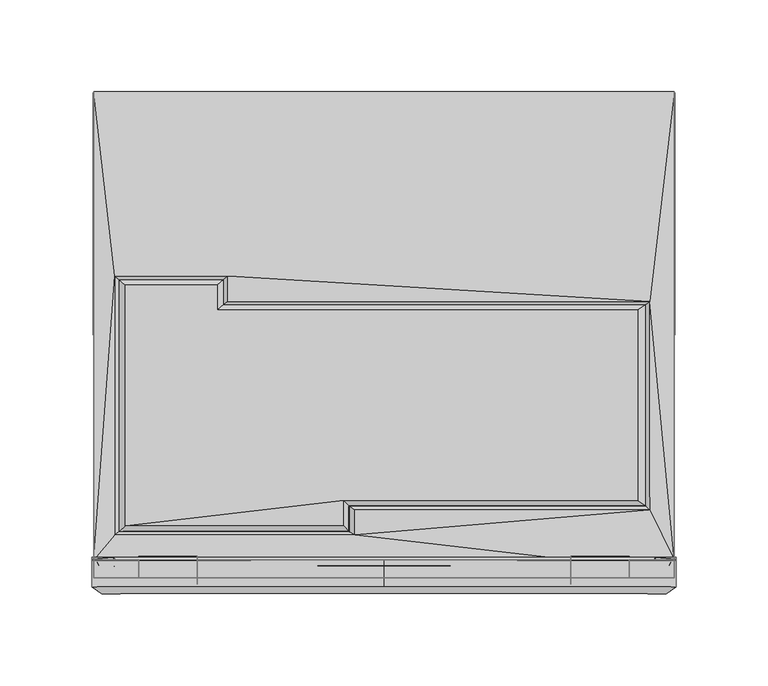
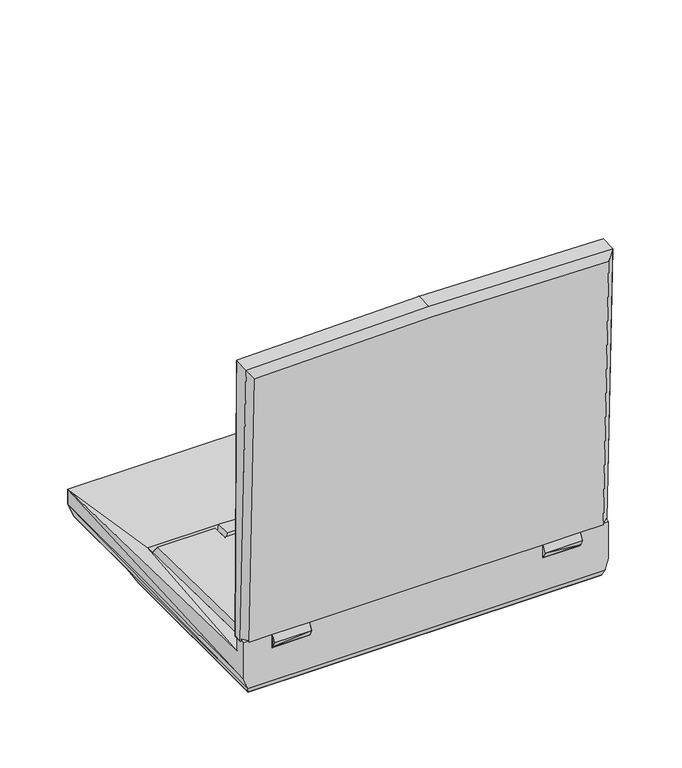
"""IFC4 building model written with IfcOpenShell, lengths in millimetres: proxy geometry, Entourage_RPC_Notebook_Computer : Entourage_RPC_Notebook_Computer."""

from ifc_helpers import new_model, si_unit, origin, place, context, project, spatial, triangles, source, transform, mapped, element, save


def entourage_8896f287(model_context):
    return source(origin(), model_context, "Body", "Tessellation", [
        triangles([(158.4296647, 167.5812681, 28.2218875), (101.7496669, -97.7313983, 35.1332139), (101.7496669, -97.7313983, 48.4910491), (101.7496669, -92.7961799, 50.2665039), (101.7496669, -87.9168539, 48.1837095), (101.7496669, -87.9168539, 35.1332139), (158.4296647, -87.9168539, 35.1332139), (133.8221823, -97.7288549, 35.1332139), (133.8221823, -97.7313983, 48.4910491), (133.8221823, -92.7961799, 50.2665039), (133.8221823, -87.9168539, 48.1837095), (133.8221823, -87.9168539, 35.1332139), (-158.4322081, 167.5812681, 28.2218875), (-101.7496669, -97.7313983, 35.1332139), (-101.7496669, -97.7313983, 48.4910491), (-101.7496669, -92.7961799, 50.2665039), (-101.7496669, -87.9168539, 48.1837095), (-101.7496669, -87.9168539, 35.1332139), (-85.2320795, 66.8399745, 31.8083601), (144.8813274, 53.1646373, 31.9658404), (-85.2320795, 53.1646373, 31.9658404), (144.8813274, -60.6703247, 34.190875), (-146.9209376, -74.3380406, 34.2924744), (-146.9209376, 66.8399745, 31.8083601), (-158.4322081, -87.9168539, 35.1332139), (-133.8247257, -97.7313983, 35.1332139), (-133.8247257, -97.7313983, 48.4910491), (-133.8247257, -92.7961799, 50.2665039), (-133.8247257, -87.9168539, 48.1837095), (-133.8247257, -87.9168539, 35.1332139), (142.7070869, -58.4935499, 29.3902845), (-15.8851303, -74.3380406, 34.2924744), (-19.0347234, -72.5752803, 29.491884), (-15.8851303, -60.6703247, 34.190875), (-19.0347234, -58.4935499, 29.3902845), (155.2851437, 164.0506697, 4.7853507), (155.2851437, 83.3296248, 4.869171), (153.4715916, 69.0040502, 0.0), (153.4715916, -95.8771965, 0.0), (-155.2876871, 164.0506697, 4.7853507), (-155.2851437, 83.3296248, 4.869171), (-153.4715916, 69.0040502, 0.0), (-153.4715916, -95.8771965, 0.0), (155.2851437, -97.7313983, 4.869171), (158.4296647, -97.7313983, 14.9046918), (158.4296647, -97.7313983, 48.4910491), (-155.2851437, -97.7313983, 4.869171), (-158.4322081, -97.7313983, 14.9046918), (-158.4322081, -97.7313983, 48.4910491), (158.4296647, -92.7961799, 50.2665039), (158.4296647, -87.9168539, 48.1837095), (-158.4322081, -92.7961799, 50.2665039), (-158.4322081, -87.9168539, 48.1837095), (158.6201509, 166.809095, 14.9046918), (-158.6201509, 166.809095, 14.9046918), (-87.4063109, 64.9654568, 27.0992089), (142.7070869, 51.2901242, 27.2541481), (-87.4063109, 51.2901242, 27.2541481), (-144.7467062, -72.5752803, 29.491884), (-144.7467062, 64.9654568, 27.0992089), (-141.2262725, 62.1181243, 32.971677), (-90.9267446, 62.1181243, 32.971677), (138.3738576, 48.4427871, 33.1266163), (-90.9267446, 48.4427871, 33.1266163), (138.3738576, -55.455713, 35.1128935), (-141.2262725, -69.5374479, 35.2170342), (-21.8820582, -55.455713, 35.1128935), (-21.8820582, -69.5374479, 35.2170342), (0.0, -90.1722394, 56.3506665), (0.0, -94.0301344, 283.6618462), (145.6915886, -90.167307, 56.3494402), (145.6915886, -94.0301344, 283.6618462), (-145.109929, -90.167307, 56.3494402), (-145.109929, -94.0301344, 283.6618462), (0.0, -86.6469732, 54.9193722), (0.0, -90.9261269, 284.9821508), (147.9064607, -86.6414321, 54.9206076), (147.9064607, -90.9261269, 284.9821508), (-147.3248011, -86.6414321, 54.9206076), (-147.3248011, -90.9261269, 284.9821508), (0.0, -88.1607071, 305.3969839), (0.0, -102.413053, 304.8563192), (159.4431202, -88.386847, 302.5685955), (159.4431202, -102.6416636, 302.0285485), (-159.4431202, -88.386847, 302.5685955), (-159.4431202, -102.6416636, 302.0285485), (0.0, -106.3485413, 297.4293198), (0.0, -98.2380444, 47.5817886), (101.7496669, -99.2864996, 36.8041307), (154.0176883, -106.5746903, 294.6009314), (101.7496669, -98.2380444, 47.5817886), (133.8221823, -99.2729467, 36.8059883), (133.7332887, -98.2380444, 47.5817886), (154.0176883, -98.2380444, 47.5817886), (133.8221823, -101.2159331, 41.6751679), (101.7496669, -101.2159331, 41.6751679), (159.4431202, -94.0607739, 47.7261203), (-101.7496669, -99.2864996, 36.8041307), (-154.0176883, -106.5746903, 294.6009314), (-101.7496669, -98.2380444, 47.5817886), (-133.8221823, -99.2729467, 36.8059883), (-133.7332887, -98.2380444, 47.5817886), (-154.0176883, -98.2380444, 47.5817886), (-133.8221823, -101.2159331, 41.6751679), (-101.7496669, -101.2159331, 41.6751679), (-159.4431202, -94.0607739, 47.7261203), (0.0, -86.4984357, 47.9871781), (101.7496669, -85.924897, 37.2684533), (101.7496669, -86.5033682, 47.9884044), (133.8221823, -85.924897, 37.2684533), (-101.7496669, -85.924897, 37.2684533), (-101.7496669, -86.5033682, 47.9884044), (-133.8221823, -85.924897, 37.2684533), (133.7332887, -86.5033682, 47.9884044), (159.4431202, -86.4953563, 47.9890267), (-133.7332887, -86.5033682, 47.9884044), (-159.4431202, -86.4953563, 47.9890267), (0.0, -88.1641952, 303.1256291), (156.9437634, -88.3928059, 300.2978765), (159.4431202, -87.6648889, 205.2385081), (0.0, -91.14827, 301.1419566), (155.5010462, -91.376263, 298.3166385), (-156.9437634, -88.3928059, 300.2978765), (-159.4431202, -87.6648889, 205.2385081), (-155.5010462, -91.376263, 298.3166385)], [[19, 1, 13], [2, 6, 3], [3, 6, 4], [4, 6, 5], [12, 6, 8], [8, 6, 2], [11, 12, 10], [10, 12, 9], [9, 12, 8], [21, 20, 19], [20, 1, 19], [22, 6, 12], [1, 20, 7], [22, 12, 7], [23, 6, 32], [18, 6, 23], [19, 13, 24], [14, 15, 18], [15, 16, 18], [16, 17, 18], [30, 26, 18], [26, 14, 18], [29, 28, 30], [28, 27, 30], [27, 26, 30], [24, 25, 23], [23, 30, 18], [13, 25, 24], [23, 25, 30], [32, 6, 22], [22, 34, 32], [31, 33, 35], [37, 41, 36], [36, 41, 40], [42, 41, 38], [38, 41, 37], [39, 43, 38], [38, 43, 42], [44, 8, 2], [8, 44, 45], [45, 46, 9], [9, 8, 45], [44, 47, 39], [39, 47, 43], [2, 14, 47], [2, 47, 44], [3, 15, 14], [3, 14, 2], [47, 14, 26], [26, 48, 47], [48, 27, 49], [27, 48, 26], [50, 51, 11], [11, 10, 50], [5, 17, 16], [5, 16, 4], [52, 29, 53], [29, 52, 28], [46, 50, 10], [10, 9, 46], [4, 16, 15], [4, 15, 3], [49, 28, 52], [28, 49, 27], [13, 1, 55], [55, 1, 54], [55, 54, 40], [40, 54, 36], [55, 40, 41], [48, 52, 25], [52, 48, 49], [53, 25, 52], [41, 43, 47], [13, 48, 25], [55, 47, 48], [43, 41, 42], [48, 13, 55], [47, 55, 41], [51, 7, 12], [12, 11, 51], [6, 18, 17], [6, 17, 5], [53, 30, 25], [30, 53, 29], [54, 37, 36], [45, 7, 50], [50, 46, 45], [51, 50, 7], [37, 44, 39], [1, 7, 45], [54, 45, 44], [39, 38, 37], [45, 54, 1], [44, 37, 54], [57, 31, 22], [23, 32, 33], [33, 59, 23], [20, 21, 58], [58, 57, 20], [21, 19, 56], [56, 58, 21], [19, 24, 60], [60, 56, 19], [24, 23, 59], [59, 60, 24], [34, 22, 31], [31, 35, 34], [33, 32, 34], [34, 35, 33], [59, 35, 33], [20, 22, 7], [22, 20, 57], [67, 65, 63], [67, 63, 64], [64, 62, 61], [66, 64, 61], [31, 57, 63], [63, 65, 31], [35, 31, 65], [65, 67, 35], [57, 58, 64], [64, 63, 57], [58, 56, 62], [62, 64, 58], [56, 60, 61], [61, 62, 56], [60, 59, 66], [66, 61, 60], [66, 67, 64], [68, 66, 59], [59, 33, 68], [35, 67, 68], [68, 33, 35], [66, 68, 67], [69, 70, 72], [69, 72, 71], [69, 74, 70], [69, 73, 74], [76, 78, 72], [72, 70, 76], [77, 75, 69], [69, 71, 77], [78, 77, 71], [71, 72, 78], [76, 74, 80], [74, 76, 70], [79, 69, 75], [69, 79, 73], [80, 73, 79], [73, 80, 74], [81, 82, 84], [81, 84, 83], [81, 86, 82], [81, 85, 86], [82, 87, 90], [82, 90, 84], [87, 88, 91], [87, 91, 90], [90, 91, 93], [96, 89, 92], [96, 92, 95], [90, 93, 94], [97, 90, 94], [91, 95, 93], [91, 96, 95], [97, 84, 90], [82, 99, 87], [82, 86, 99], [87, 100, 88], [87, 99, 100], [99, 102, 100], [105, 101, 98], [105, 104, 101], [102, 99, 103], [106, 103, 99], [100, 102, 104], [100, 104, 105], [106, 99, 86], [89, 108, 110], [89, 110, 92], [96, 91, 89], [89, 91, 108], [108, 91, 109], [91, 88, 109], [109, 88, 107], [98, 113, 111], [98, 101, 113], [105, 98, 100], [98, 111, 100], [111, 112, 100], [100, 112, 88], [112, 107, 88], [93, 114, 115], [93, 115, 97], [95, 92, 93], [93, 92, 114], [114, 92, 110], [93, 97, 94], [102, 117, 116], [102, 106, 117], [104, 102, 101], [102, 116, 101], [116, 113, 101], [102, 103, 106], [108, 109, 114], [108, 114, 110], [81, 83, 119], [109, 107, 75], [75, 77, 109], [114, 109, 77], [120, 115, 77], [114, 77, 115], [119, 118, 81], [77, 78, 120], [119, 120, 122], [76, 121, 122], [76, 122, 78], [119, 122, 121], [119, 121, 118], [120, 78, 122], [83, 120, 119], [111, 116, 112], [111, 113, 116], [81, 123, 85], [112, 75, 107], [75, 112, 79], [116, 79, 112], [124, 79, 117], [117, 79, 116], [123, 81, 118], [79, 124, 80], [123, 125, 124], [76, 125, 121], [76, 80, 125], [123, 121, 125], [123, 118, 121], [124, 125, 80], [85, 123, 124], [117, 86, 124], [117, 106, 86], [124, 86, 85], [115, 120, 84], [115, 84, 97], [120, 83, 84]], closed=False),
    ])


if __name__ == "__main__":
    model = new_model("IFC4")
    model_context = context("Model", 3, world=origin())
    ifc_project = project(units=[si_unit("LENGTHUNIT", "METRE", prefix="MILLI")], contexts=[model_context])
    site = spatial("IfcSite", under=ifc_project)
    building = spatial("IfcBuilding", under=site)
    placement = place(None, origin())
    entourage_shape = entourage_8896f287(model_context)
    element("IfcBuildingElementProxy", 1, Name="Entourage_RPC_Notebook_Computer : Entourage_RPC_Notebook_Computer", ObjectType="Entourage_RPC_Notebook_Computer : Entourage_RPC_Notebook_Computer", at=placement, inside=building, context=model_context, shape_type="MappedRepresentation", body=[
        mapped(entourage_shape, transform((0.0, 0.0, 0.0), x_axis=(1.0, 0.0, 0.0), y_axis=(0.0, 1.0, 0.0), z_axis=(0.0, 0.0, 1.0))),
    ])
    save(model, "model.ifc")

# Revit data of these elements
# Type "Entourage_RPC_Notebook_Computer : Entourage_RPC_Notebook_Computer"
#   built-in parameter 1005198 = "{2, 15},{39, RPC-16-N04H-AQSP-D1N4-43SU-6GKQ-C3KU-1C},{1, 0},{1, 0},{2, 33},{1, 8},{5, Color},{1, 0},{1, 0},{3, 0.8},{3, 0.8},{3, 0.8},{1, 8},{7, BBoxMin},{1, 0},{1, 0},{1, 0},{1, 0},{1, 0},{1, 8},{7, BBoxMax},{1, 0},{1, 0},{1, 0},{1, 0},{1, 0},{2, 11},{9, RPCTypeId},{1, 0},{1, 0},{39, RPC-16-N04H-AQSP-D1N4-43SU-6GKQ-C3KU-1C},{1, 6},{14, RPCPlantHeight},{1, 0},{1, 0},{7, 2.28517},{2, 11},{20, AdvancedUIDefinition},{1, 0},{1, 0},{0, },{2, 11},{10, AssetLibID},{1, 0},{1, 0},{36, 4D3F6E72-3F99-4203-98E9-AF80B3C7A7A4},{2, 11},{10, BaseSchema},{1, 0},{1, 0},{9, RPCSchema},{1, 2},{6, Hidden},{1, 0},{1, 0},{1, 0},{2, 11},{12, LocalizedUID},{1, 0},{1, 0},{0, },{1, 4},{11, RPCCategory},{1, 0},{1, 0},{1, 0},{2, 11},{8, RPCImage},{1, 0},{1, 0},{0, },{1, 4},{13, SchemaVersion},{1, 0},{1, 0},{1, 3},{2, 11},{12, UIDefinition},{1, 0},{1, 0},{0, },{2, 11},{6, UIName},{1, 0},{1, 0},{39, RPC-16-N04H-AQSP-D1N4-43SU-6GKQ-C3KU-1C},{2, 11},{11, VersionGUID},{1, 0},{1, 0},{9, RPCSchema},{2, 11},{9, assettype},{1, 0},{1, 0},{11, RPCGeometry},{2, 11},{11, description},{1, 0},{1, 0},{0, },{2, 11},{9, localname},{1, 0},{1, 0},{3, RPC},{2, 11},{9, localtype},{1, 0},{1, 0},{3, RPC},{1, 4},{8, revision},{1, 0},{1, 0},{1, 1},{2, 11},{9, thumbnail},{1, 0},{1, 0},{0, },{1, 4},{7, version},{1, 0},{1, 0},{1, 1},{2, 14},{6, Height},{1, 0},{1, 0},{7, 2.28517},{1, 2},{20, RPC_Cast Reflections},{1, 0},{1, 0},{1, 0},{1, 4},{8, RPC_Open},{1, 0},{1, 0},{3, -14},{1, 2},{9, RPC_Power},{1, 0},{1, 0},{1, 1},{2, 11},{18, RPC_Screen Preview},{1, 0},{1, 0},{70, __RPC:/object data/textures/object/Top/TopScreen/textures/on/rgb/0/0/0},{2, 11},{20, RPC_i_Screen Preview},{1, 0},{1, 0},{0, },{1, 2},{17, RPC_Custom Screen},{1, 0},{1, 0},{1, 1},{2, 11},{20, RPC_Screen File Name},{1, 0},{1, 0},{56, C:\\Users\\Mary\\Desktop\\Photos\\Brian Aug 2013\\Castle 1.jpg},{2, 11},{7, keyword},{1, 0},{1, 0},{31, :Geometry:RPC:Notebook Computer},{2, 11},{8, category},{1, 0},{1, 0},{15, :Office Clutter},{21, assetlibrary_base.fbx},{1, 5},"
#   built-in parameter 1005195 = "RPC-16-N04H-AQSP-D1N4-43SU-6GKQ-C3KU-1C"
#   Height = 0
